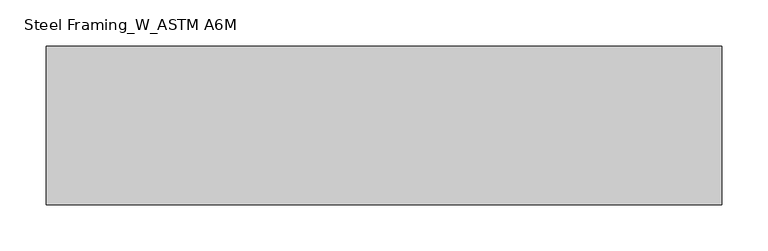
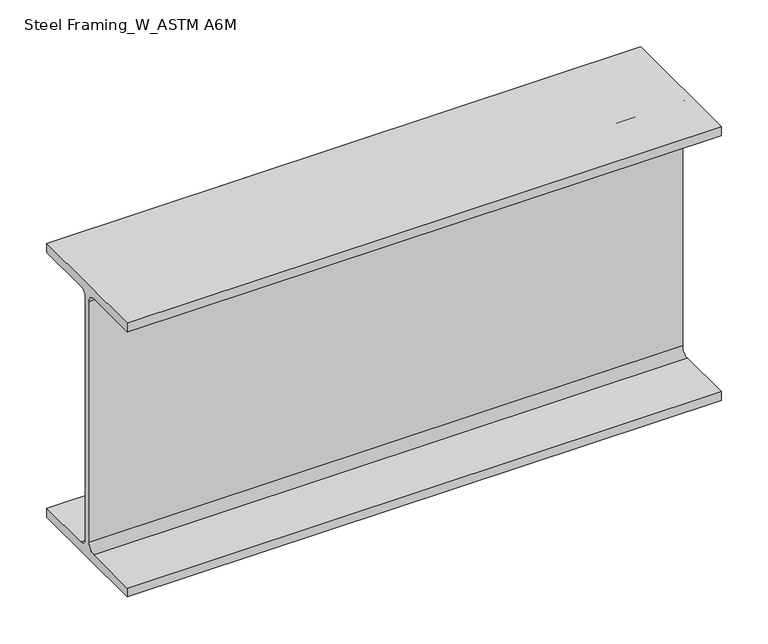
"""IFC4 building model written with IfcOpenShell, lengths in millimetres: beam geometry, Steel Framing_W_ASTM A6M : H_SB_AR_S02_W360x51_RG1."""

from ifc_helpers import new_model, si_unit, point, frame, frame_2d, origin, place, context, project, spatial, polyline, circle_curve, trimmed, segment, composite_curve, outline, extrude, source, transform, mapped, element, save


def steel_framing_w_astm_a6m_1c0913ec(model_context):
    return source(origin(), model_context, "Body", "SweptSolid", [
        extrude(outline(composite_curve([segment(polyline([(85.5, -166.4), (85.5, -178.0), (-85.5, -178.0), (-85.5, -166.4), (-13.72, -166.4)]), True, "CONTINUOUS"), segment(trimmed(circle_curve(frame_2d((-13.72, -156.3)), 10.1), [point((-13.72, -166.4))], [point((-3.62, -156.3))], True, "CARTESIAN"), True, "CONTINUOUS"), segment(polyline([(-3.62, -156.3), (-3.62, 156.3)]), True, "CONTINUOUS"), segment(trimmed(circle_curve(frame_2d((-13.72, 156.3)), 10.1), [point((-3.62, 156.3))], [point((-13.72, 166.4))], True, "CARTESIAN"), True, "CONTINUOUS"), segment(polyline([(-13.72, 166.4), (-85.5, 166.4), (-85.5, 178.0), (85.5, 178.0), (85.5, 166.4), (13.72, 166.4)]), True, "CONTINUOUS"), segment(trimmed(circle_curve(frame_2d((13.72, 156.3)), 10.1), [point((13.72, 166.4))], [point((3.62, 156.3))], True, "CARTESIAN"), True, "CONTINUOUS"), segment(polyline([(3.62, 156.3), (3.62, -156.3)]), True, "CONTINUOUS"), segment(trimmed(circle_curve(frame_2d((13.72, -156.3)), 10.1), [point((3.62, -156.3))], [point((13.72, -166.4))], True, "CARTESIAN"), True, "CONTINUOUS"), segment(polyline([(13.72, -166.4), (85.5, -166.4)]), True, "CONTINUOUS")], self_intersect=False)), frame((-480.9, 0.0, 0.0), z_axis=(1.0, 0.0, 0.0), x_axis=(0.0, 1.0, 0.0)), (0.0, 0.0, 1.0), 729.5),
    ])


if __name__ == "__main__":
    model = new_model("IFC4")
    model_context = context("Model", 3, world=origin())
    ifc_project = project(units=[si_unit("LENGTHUNIT", "METRE", prefix="MILLI")], contexts=[model_context])
    site = spatial("IfcSite", under=ifc_project)
    building = spatial("IfcBuilding", under=site)
    placement = place(None, origin())
    steel_framing_w_astm_a6m_shape = steel_framing_w_astm_a6m_1c0913ec(model_context)
    element("IfcBeam", 1, ObjectType="Steel Framing_W_ASTM A6M : H_SB_AR_S02_W360x51_RG1", at=placement, inside=building, context=model_context, shape_type="MappedRepresentation", body=[
        mapped(steel_framing_w_astm_a6m_shape, transform((0.0, 0.0, 0.0), x_axis=(1.0, 0.0, 0.0), y_axis=(0.0, 1.0, 0.0), z_axis=(0.0, 0.0, 1.0))),
    ])
    save(model, "model.ifc")

# Revit data of these elements
# Type "Steel Framing_W_ASTM A6M : H_SB_AR_S02_W360x51_RG1"
#   Type Mark = "RG1"
#   Section Name Key = "W14x34"
#   Width = 17.1 cm
#   Web Thickness = 0.724 cm
#   Web Fillet = 1.01 cm
#   Warping Constant = 287000.0 cm⁶
#   Torsional Moment of Inertia = 23.70 cm⁴
#   Section Area = 64.5 cm²
#   Plastic Modulus weak axis = 174.0 cm³
#   Plastic Modulus strong axis = 895.0 cm³
#   Perimeter = 1.36 m²/m
#   Nominal Weight = 51.00 kgf/m
#   Moment of Inertia weak axis = 970.00 cm⁴
#   Moment of Inertia strong axis = 14200.00 cm⁴
#   Height = 35.6 cm
#   Flange Thickness = 1.16 cm
#   Elastic Modulus weak axis = 113.0 cm³
#   Elastic Modulus strong axis = 796.0 cm³
#   Centroid Vertical = 17.8 cm
#   Centroid Horizontal = 8.55 cm
#   Length [instance default] = 1500 mm
#   Structural Material [instance default] = Steel, 45-345
#   Bolt Spacing = 0
#   Assembly Code = ""
# Element 1 (IfcBeam, "Steel Framing_W_ASTM A6M : H_SB_AR_S02_W360x51_RG1")
#   Materials on its faces: "Steel, 45-345"
# Materials
#   "Steel, 45-345": class "Metal", colour RGB 189 187 185, transparency 0, Description = "Steel 345 MPa", Cost = 0
